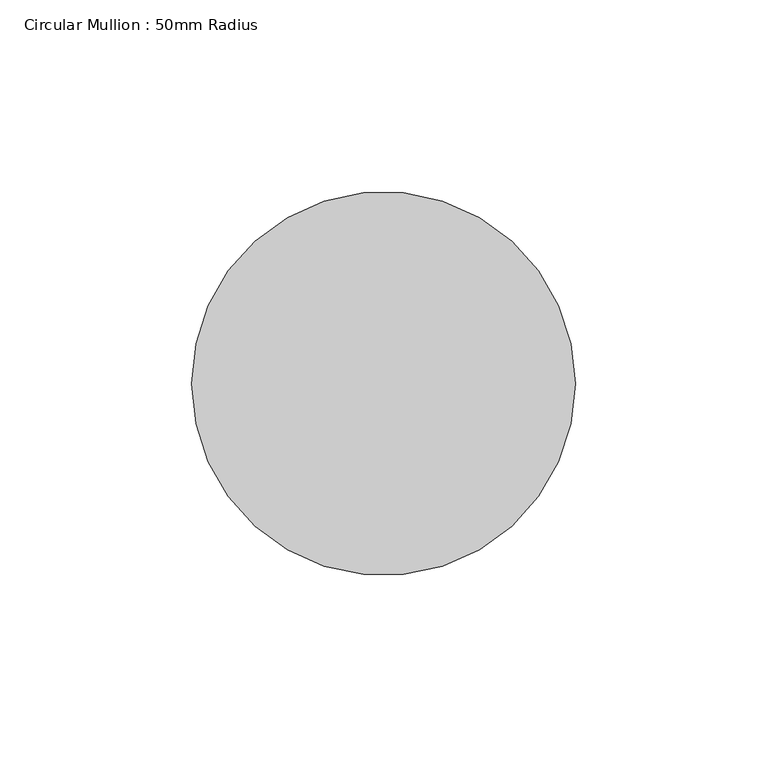
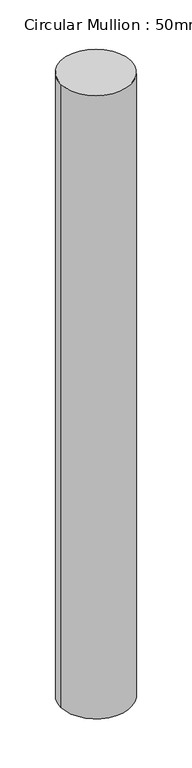
"""IFC4 building model written with IfcOpenShell, lengths in millimetres: member geometry, Circular Mullion : 50mm Radius."""

import ifcopenshell
import ifcopenshell.guid

model = None  # the IFC model being written
_history = None  # IfcOwnerHistory: only IFC2X3 demands one
_inside = {}  # id of a spatial element -> (the spatial element, [elements in it])
_under = {}  # id of a project, library or spatial element -> (it, [spatial elements below it])
_declared = {}  # id of a project -> (the project, [libraries it declares])
_typed = {}  # id of a type object -> (the type object, [elements of that type])
_made_of = {}  # id of a material, layer set ... -> (it, [elements and type objects made of it])


def new_model(schema):
    """Start an empty IFC model of exactly this schema.

    Asked for "IFC4X3", IfcOpenShell would pick the latest addendum, in which some entities
    have other attributes; the version numbers below select the first issue.
    IFC2X3 requires an IfcOwnerHistory on every rooted entity: one is made here for all.
    """
    global model, _history
    if schema == "IFC4X3":
        model = ifcopenshell.file(schema_version=(4, 3, 0, 0))
    else:
        model = ifcopenshell.file(schema=schema)
    _inside.clear()
    _under.clear()
    _declared.clear()
    _typed.clear()
    _made_of.clear()
    _history = None
    if model.schema == "IFC2X3":
        org = make("IfcOrganization", Name="unknown")
        user = make(
            "IfcPersonAndOrganization",
            ThePerson=make("IfcPerson", FamilyName="unknown"),
            TheOrganization=org,
        )
        app = make(
            "IfcApplication",
            ApplicationDeveloper=org,
            Version="unknown",
            ApplicationFullName="unknown",
            ApplicationIdentifier="unknown",
        )
        _history = make(
            "IfcOwnerHistory",
            OwningUser=user,
            OwningApplication=app,
            ChangeAction="ADDED",
            CreationDate=0,
        )
    return model


def make(cls, **values):
    """One entity of the class cls with the attributes given. An attribute that is None is left unset."""
    return model.create_entity(
        cls, **{name: value for name, value in values.items() if value is not None}
    )


def rooted(cls, **values):
    """An entity with a GlobalId (a new one), such as an element, a storey or a relation."""
    return make(cls, GlobalId=ifcopenshell.guid.new(), OwnerHistory=_history, **values)


def si_unit(unit_type, name, prefix=None):
    """IfcSIUnit, for example si_unit("LENGTHUNIT", "METRE", prefix="MILLI")."""
    return make("IfcSIUnit", UnitType=unit_type, Prefix=prefix, Name=name)


def assignment(units):
    """IfcUnitAssignment: the units of a project."""
    return None if units is None else make("IfcUnitAssignment", Units=units)


def point(xyz):
    """IfcCartesianPoint."""
    return None if xyz is None else make("IfcCartesianPoint", Coordinates=xyz)


def direction(xyz):
    """IfcDirection."""
    return None if xyz is None else make("IfcDirection", DirectionRatios=xyz)


def frame(location, z_axis=None, x_axis=None):
    """IfcAxis2Placement3D, a coordinate frame: its origin and axes. An axis left out is left unset."""
    return make(
        "IfcAxis2Placement3D",
        Location=point(location),
        Axis=direction(z_axis),
        RefDirection=direction(x_axis),
    )


def frame_2d(location, x_axis=None):
    """IfcAxis2Placement2D, a coordinate frame in the plane: its origin and x axis."""
    return make(
        "IfcAxis2Placement2D", Location=point(location), RefDirection=direction(x_axis)
    )


def origin():
    """The frame at (0, 0, 0) with its axes left unset."""
    return frame((0.0, 0.0, 0.0))


def origin_2d():
    """The frame at (0, 0) in the plane with its x axis left unset."""
    return frame_2d((0.0, 0.0))


def place(relative_to, where):
    """IfcLocalPlacement: puts the frame where relative to a parent placement (None: the world)."""
    return make(
        "IfcLocalPlacement", PlacementRelTo=relative_to, RelativePlacement=where
    )


def context(
    kind, dimensions, precision=None, world=None, true_north=None, identifier=None
):
    """IfcGeometricRepresentationContext, for example the 3D "Model" context."""
    return make(
        "IfcGeometricRepresentationContext",
        ContextIdentifier=identifier,
        ContextType=kind,
        CoordinateSpaceDimension=dimensions,
        Precision=precision,
        WorldCoordinateSystem=world,
        TrueNorth=true_north,
    )


def project(units=None, contexts=None):
    """IfcProject with its units and contexts."""
    return rooted(
        "IfcProject",
        Name="project",
        RepresentationContexts=contexts,
        UnitsInContext=assignment(units),
    )


def spatial(cls, under=None, at=None, **own):
    """A site, building, storey or space (cls), placed at a placement, below another one or the project."""
    s = rooted(cls, ObjectPlacement=at, **own)
    if under is not None:
        _under.setdefault(under.id(), (under, []))[1].append(s)
    return s


def circle_curve(where, radius):
    """IfcCircle in the frame where."""
    return make("IfcCircle", Position=where, Radius=radius)


def trimmed(basis, trim1, trim2, sense, master):
    """IfcTrimmedCurve: the piece of a basis curve between two trims."""
    return make(
        "IfcTrimmedCurve",
        BasisCurve=basis,
        Trim1=trim1,
        Trim2=trim2,
        SenseAgreement=sense,
        MasterRepresentation=master,
    )


def segment(curve, same_sense, transition):
    """IfcCompositeCurveSegment."""
    return make(
        "IfcCompositeCurveSegment",
        Transition=transition,
        SameSense=same_sense,
        ParentCurve=curve,
    )


def composite_curve(segments, self_intersect=None):
    """IfcCompositeCurve: segments joined end to end."""
    return make("IfcCompositeCurve", Segments=segments, SelfIntersect=self_intersect)


def outline(outer, holes=None, kind="AREA"):
    """IfcArbitraryClosedProfileDef: a profile drawn as a closed curve; with holes, ...WithVoids."""
    if holes is None:
        return make("IfcArbitraryClosedProfileDef", ProfileType=kind, OuterCurve=outer)
    return make(
        "IfcArbitraryProfileDefWithVoids",
        ProfileType=kind,
        OuterCurve=outer,
        InnerCurves=holes,
    )


def extrude(swept, where, along, depth):
    """IfcExtrudedAreaSolid: the profile swept, set in the frame where, extruded along a direction by depth."""
    return make(
        "IfcExtrudedAreaSolid",
        SweptArea=swept,
        Position=where,
        ExtrudedDirection=direction(along),
        Depth=depth,
    )


def shape(context_of_items, identifier, shape_type, items):
    """IfcShapeRepresentation: the items that make up one representation, for example the "Body"."""
    return make(
        "IfcShapeRepresentation",
        ContextOfItems=context_of_items,
        RepresentationIdentifier=identifier,
        RepresentationType=shape_type,
        Items=items,
    )


def source(mapping_origin, context_of_items, identifier, shape_type, items):
    """IfcRepresentationMap: a shape defined once, which mapped items show again and again."""
    return make(
        "IfcRepresentationMap",
        MappingOrigin=mapping_origin,
        MappedRepresentation=shape(context_of_items, identifier, shape_type, items),
    )


def transform(
    local_origin,
    x_axis=None,
    y_axis=None,
    z_axis=None,
    scale=None,
    scale2=None,
    scale3=None,
    uniform=True,
):
    """IfcCartesianTransformationOperator3D, or its non-uniform kind. x_axis, y_axis, z_axis: its Axis1, 2, 3."""
    if uniform:
        return make(
            "IfcCartesianTransformationOperator3D",
            Axis1=direction(x_axis),
            Axis2=direction(y_axis),
            LocalOrigin=point(local_origin),
            Scale=scale,
            Axis3=direction(z_axis),
        )
    return make(
        "IfcCartesianTransformationOperator3DnonUniform",
        Axis1=direction(x_axis),
        Axis2=direction(y_axis),
        LocalOrigin=point(local_origin),
        Scale=scale,
        Axis3=direction(z_axis),
        Scale2=scale2,
        Scale3=scale3,
    )


def mapped(mapping_source, mapping_target):
    """IfcMappedItem: shows the shape of a source again, moved by a transform."""
    return make(
        "IfcMappedItem", MappingSource=mapping_source, MappingTarget=mapping_target
    )


def made_of(thing, what):
    """Note that an element or type object is made of a material, layer set ...; save() writes the relation."""
    if what is not None:
        _made_of.setdefault(what.id(), (what, []))[1].append(thing)
    return thing


def element(
    cls,
    number,
    at=None,
    inside=None,
    cuts=None,
    type_object=None,
    material=None,
    context=None,
    identifier="Body",
    shape_type=None,
    held_by="IfcProductDefinitionShape",
    body=None,
    shapes=None,
    **own,
):
    """One element of the class cls, such as IfcWall. Its Tag is "e" and its number.

    at: its placement. inside: the storey or other place that contains it. cuts: it is an
    opening in that element (IfcRelVoidsElement). A single representation is given by context,
    identifier, shape_type and body (its items); several are given by shapes. held_by: the class
    of the entity that holds the representations. save() writes the other relations.
    """
    e = rooted(cls, Tag="e%d" % number, ObjectPlacement=at, **own)
    if body is not None:
        shapes = [shape(context, identifier, shape_type, body)]
    if shapes is not None:
        e.Representation = make(held_by, Representations=shapes)
    if inside is not None:
        _inside.setdefault(inside.id(), (inside, []))[1].append(e)
    if cuts is not None:
        rooted(
            "IfcRelVoidsElement", RelatingBuildingElement=cuts, RelatedOpeningElement=e
        )
    if type_object is not None:
        _typed.setdefault(type_object.id(), (type_object, []))[1].append(e)
    return made_of(e, material)


def aggregate(whole, parts):
    """IfcRelAggregates: a whole, such as a stair, and the parts it consists of."""
    return rooted("IfcRelAggregates", RelatingObject=whole, RelatedObjects=parts)


def save(model, path):
    """Write the relations noted so far, then the file.

    IfcRelAggregates (storeys below a building ...), IfcRelContainedInSpatialStructure (elements
    in a storey), IfcRelDefinesByType, IfcRelAssociatesMaterial and IfcRelDeclares: one each for
    every whole, place, type object, material and project.
    """
    for whole, parts in _under.values():
        aggregate(whole, parts)
    for where, things in _inside.values():
        rooted(
            "IfcRelContainedInSpatialStructure",
            RelatedElements=things,
            RelatingStructure=where,
        )
    for kind, things in _typed.values():
        rooted("IfcRelDefinesByType", RelatedObjects=things, RelatingType=kind)
    for what, things in _made_of.values():
        rooted("IfcRelAssociatesMaterial", RelatedObjects=things, RelatingMaterial=what)
    for by, libraries in _declared.values():
        rooted("IfcRelDeclares", RelatingContext=by, RelatedDefinitions=libraries)
    model.write(path)


def circular_mullion_50mm_radius_80885254(model_context):
    return source(origin(), model_context, "Body", "SweptSolid", [
        extrude(outline(composite_curve([segment(trimmed(circle_curve(origin_2d(), 50.0), [point((50.0, 0.0))], [point((-50.0, 0.0))], False, "CARTESIAN"), True, "CONTINUOUS"), segment(trimmed(circle_curve(origin_2d(), 50.0), [point((-50.0, 0.0))], [point((50.0, 0.0))], False, "CARTESIAN"), True, "CONTINUOUS")], self_intersect=False)), frame((0.0, 0.0, -937.0655689), z_axis=(0.0, 0.0, 1.0), x_axis=(1.0, 0.0, 0.0)), (0.0, 0.0, 1.0), 937.0655689),
    ])


if __name__ == "__main__":
    model = new_model("IFC4")
    model_context = context("Model", 3, world=origin())
    ifc_project = project(units=[si_unit("LENGTHUNIT", "METRE", prefix="MILLI")], contexts=[model_context])
    site = spatial("IfcSite", under=ifc_project)
    building = spatial("IfcBuilding", under=site)
    placement = place(None, origin())
    circular_mullion_50mm_radius_shape = circular_mullion_50mm_radius_80885254(model_context)
    element("IfcMember", 1, ObjectType="Circular Mullion : 50mm Radius", at=placement, inside=building, context=model_context, shape_type="MappedRepresentation", body=[
        mapped(circular_mullion_50mm_radius_shape, transform((0.0, 0.0, 0.0), x_axis=(1.0, 0.0, 0.0), y_axis=(0.0, 1.0, 0.0), z_axis=(0.0, 0.0, 1.0))),
    ])
    save(model, "model.ifc")

# Revit data of these elements
# Type "Circular Mullion : 50mm Radius"
#   built-in parameter 1007350 = 0.164042 (stored number, unit not read)
# Element 1 (IfcMember, "Circular Mullion : 50mm Radius")
#   Materials on its faces: "Aluminium"
# Materials
#   "Aluminium": class "Metal", colour RGB 247 247 247, transparency 0, Description = "Aluminium 6061", Cost = 0
